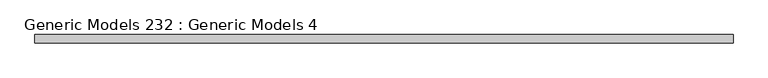
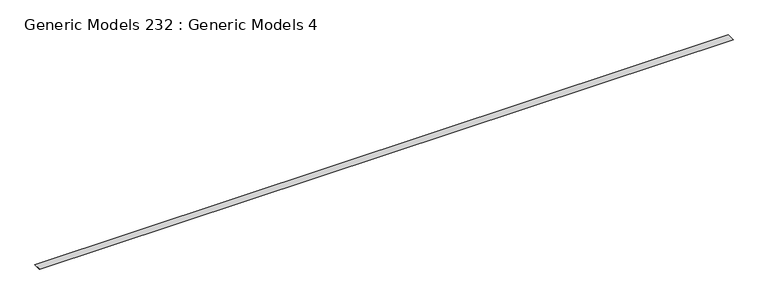
"""IFC4 building model written with IfcOpenShell, lengths in millimetres: proxy geometry, Generic Models 232 : Generic Models 4."""

import ifcopenshell
import ifcopenshell.guid

model = None  # the IFC model being written
_history = None  # IfcOwnerHistory: only IFC2X3 demands one
_inside = {}  # id of a spatial element -> (the spatial element, [elements in it])
_under = {}  # id of a project, library or spatial element -> (it, [spatial elements below it])
_declared = {}  # id of a project -> (the project, [libraries it declares])
_typed = {}  # id of a type object -> (the type object, [elements of that type])
_made_of = {}  # id of a material, layer set ... -> (it, [elements and type objects made of it])


def new_model(schema):
    """Start an empty IFC model of exactly this schema.

    Asked for "IFC4X3", IfcOpenShell would pick the latest addendum, in which some entities
    have other attributes; the version numbers below select the first issue.
    IFC2X3 requires an IfcOwnerHistory on every rooted entity: one is made here for all.
    """
    global model, _history
    if schema == "IFC4X3":
        model = ifcopenshell.file(schema_version=(4, 3, 0, 0))
    else:
        model = ifcopenshell.file(schema=schema)
    _inside.clear()
    _under.clear()
    _declared.clear()
    _typed.clear()
    _made_of.clear()
    _history = None
    if model.schema == "IFC2X3":
        org = make("IfcOrganization", Name="unknown")
        user = make(
            "IfcPersonAndOrganization",
            ThePerson=make("IfcPerson", FamilyName="unknown"),
            TheOrganization=org,
        )
        app = make(
            "IfcApplication",
            ApplicationDeveloper=org,
            Version="unknown",
            ApplicationFullName="unknown",
            ApplicationIdentifier="unknown",
        )
        _history = make(
            "IfcOwnerHistory",
            OwningUser=user,
            OwningApplication=app,
            ChangeAction="ADDED",
            CreationDate=0,
        )
    return model


def make(cls, **values):
    """One entity of the class cls with the attributes given. An attribute that is None is left unset."""
    return model.create_entity(
        cls, **{name: value for name, value in values.items() if value is not None}
    )


def rooted(cls, **values):
    """An entity with a GlobalId (a new one), such as an element, a storey or a relation."""
    return make(cls, GlobalId=ifcopenshell.guid.new(), OwnerHistory=_history, **values)


def si_unit(unit_type, name, prefix=None):
    """IfcSIUnit, for example si_unit("LENGTHUNIT", "METRE", prefix="MILLI")."""
    return make("IfcSIUnit", UnitType=unit_type, Prefix=prefix, Name=name)


def assignment(units):
    """IfcUnitAssignment: the units of a project."""
    return None if units is None else make("IfcUnitAssignment", Units=units)


def point(xyz):
    """IfcCartesianPoint."""
    return None if xyz is None else make("IfcCartesianPoint", Coordinates=xyz)


def direction(xyz):
    """IfcDirection."""
    return None if xyz is None else make("IfcDirection", DirectionRatios=xyz)


def frame(location, z_axis=None, x_axis=None):
    """IfcAxis2Placement3D, a coordinate frame: its origin and axes. An axis left out is left unset."""
    return make(
        "IfcAxis2Placement3D",
        Location=point(location),
        Axis=direction(z_axis),
        RefDirection=direction(x_axis),
    )


def origin():
    """The frame at (0, 0, 0) with its axes left unset."""
    return frame((0.0, 0.0, 0.0))


def place(relative_to, where):
    """IfcLocalPlacement: puts the frame where relative to a parent placement (None: the world)."""
    return make(
        "IfcLocalPlacement", PlacementRelTo=relative_to, RelativePlacement=where
    )


def context(
    kind, dimensions, precision=None, world=None, true_north=None, identifier=None
):
    """IfcGeometricRepresentationContext, for example the 3D "Model" context."""
    return make(
        "IfcGeometricRepresentationContext",
        ContextIdentifier=identifier,
        ContextType=kind,
        CoordinateSpaceDimension=dimensions,
        Precision=precision,
        WorldCoordinateSystem=world,
        TrueNorth=true_north,
    )


def project(units=None, contexts=None):
    """IfcProject with its units and contexts."""
    return rooted(
        "IfcProject",
        Name="project",
        RepresentationContexts=contexts,
        UnitsInContext=assignment(units),
    )


def spatial(cls, under=None, at=None, **own):
    """A site, building, storey or space (cls), placed at a placement, below another one or the project."""
    s = rooted(cls, ObjectPlacement=at, **own)
    if under is not None:
        _under.setdefault(under.id(), (under, []))[1].append(s)
    return s


def polyline(points):
    """IfcPolyline through the points."""
    return make("IfcPolyline", Points=[point(p) for p in points])


def outline(outer, holes=None, kind="AREA"):
    """IfcArbitraryClosedProfileDef: a profile drawn as a closed curve; with holes, ...WithVoids."""
    if holes is None:
        return make("IfcArbitraryClosedProfileDef", ProfileType=kind, OuterCurve=outer)
    return make(
        "IfcArbitraryProfileDefWithVoids",
        ProfileType=kind,
        OuterCurve=outer,
        InnerCurves=holes,
    )


def extrude(swept, where, along, depth):
    """IfcExtrudedAreaSolid: the profile swept, set in the frame where, extruded along a direction by depth."""
    return make(
        "IfcExtrudedAreaSolid",
        SweptArea=swept,
        Position=where,
        ExtrudedDirection=direction(along),
        Depth=depth,
    )


def shape(context_of_items, identifier, shape_type, items):
    """IfcShapeRepresentation: the items that make up one representation, for example the "Body"."""
    return make(
        "IfcShapeRepresentation",
        ContextOfItems=context_of_items,
        RepresentationIdentifier=identifier,
        RepresentationType=shape_type,
        Items=items,
    )


def source(mapping_origin, context_of_items, identifier, shape_type, items):
    """IfcRepresentationMap: a shape defined once, which mapped items show again and again."""
    return make(
        "IfcRepresentationMap",
        MappingOrigin=mapping_origin,
        MappedRepresentation=shape(context_of_items, identifier, shape_type, items),
    )


def transform(
    local_origin,
    x_axis=None,
    y_axis=None,
    z_axis=None,
    scale=None,
    scale2=None,
    scale3=None,
    uniform=True,
):
    """IfcCartesianTransformationOperator3D, or its non-uniform kind. x_axis, y_axis, z_axis: its Axis1, 2, 3."""
    if uniform:
        return make(
            "IfcCartesianTransformationOperator3D",
            Axis1=direction(x_axis),
            Axis2=direction(y_axis),
            LocalOrigin=point(local_origin),
            Scale=scale,
            Axis3=direction(z_axis),
        )
    return make(
        "IfcCartesianTransformationOperator3DnonUniform",
        Axis1=direction(x_axis),
        Axis2=direction(y_axis),
        LocalOrigin=point(local_origin),
        Scale=scale,
        Axis3=direction(z_axis),
        Scale2=scale2,
        Scale3=scale3,
    )


def mapped(mapping_source, mapping_target):
    """IfcMappedItem: shows the shape of a source again, moved by a transform."""
    return make(
        "IfcMappedItem", MappingSource=mapping_source, MappingTarget=mapping_target
    )


def made_of(thing, what):
    """Note that an element or type object is made of a material, layer set ...; save() writes the relation."""
    if what is not None:
        _made_of.setdefault(what.id(), (what, []))[1].append(thing)
    return thing


def element(
    cls,
    number,
    at=None,
    inside=None,
    cuts=None,
    type_object=None,
    material=None,
    context=None,
    identifier="Body",
    shape_type=None,
    held_by="IfcProductDefinitionShape",
    body=None,
    shapes=None,
    **own,
):
    """One element of the class cls, such as IfcWall. Its Tag is "e" and its number.

    at: its placement. inside: the storey or other place that contains it. cuts: it is an
    opening in that element (IfcRelVoidsElement). A single representation is given by context,
    identifier, shape_type and body (its items); several are given by shapes. held_by: the class
    of the entity that holds the representations. save() writes the other relations.
    """
    e = rooted(cls, Tag="e%d" % number, ObjectPlacement=at, **own)
    if body is not None:
        shapes = [shape(context, identifier, shape_type, body)]
    if shapes is not None:
        e.Representation = make(held_by, Representations=shapes)
    if inside is not None:
        _inside.setdefault(inside.id(), (inside, []))[1].append(e)
    if cuts is not None:
        rooted(
            "IfcRelVoidsElement", RelatingBuildingElement=cuts, RelatedOpeningElement=e
        )
    if type_object is not None:
        _typed.setdefault(type_object.id(), (type_object, []))[1].append(e)
    return made_of(e, material)


def aggregate(whole, parts):
    """IfcRelAggregates: a whole, such as a stair, and the parts it consists of."""
    return rooted("IfcRelAggregates", RelatingObject=whole, RelatedObjects=parts)


def save(model, path):
    """Write the relations noted so far, then the file.

    IfcRelAggregates (storeys below a building ...), IfcRelContainedInSpatialStructure (elements
    in a storey), IfcRelDefinesByType, IfcRelAssociatesMaterial and IfcRelDeclares: one each for
    every whole, place, type object, material and project.
    """
    for whole, parts in _under.values():
        aggregate(whole, parts)
    for where, things in _inside.values():
        rooted(
            "IfcRelContainedInSpatialStructure",
            RelatedElements=things,
            RelatingStructure=where,
        )
    for kind, things in _typed.values():
        rooted("IfcRelDefinesByType", RelatedObjects=things, RelatingType=kind)
    for what, things in _made_of.values():
        rooted("IfcRelAssociatesMaterial", RelatedObjects=things, RelatingMaterial=what)
    for by, libraries in _declared.values():
        rooted("IfcRelDeclares", RelatingContext=by, RelatedDefinitions=libraries)
    model.write(path)


def generic_models_232_generic_models_4_c391f1b5(model_context):
    return source(origin(), model_context, "Body", "SweptSolid", [
        extrude(outline(polyline([(11796.8702948, 127086.238344), (11763.5680231, 127103.3395105), (11988.322106, 127107.9460991), (11952.2508948, 127089.4230447), (11796.8702948, 127086.238344)])), frame((-10234.5171316, 0.0, 0.0), z_axis=(1.0, 0.0, 0.0), x_axis=(0.0, 1.0, 0.0)), (0.0, 0.0, 1.0), 18643.6),
    ])


if __name__ == "__main__":
    model = new_model("IFC4")
    model_context = context("Model", 3, world=origin())
    ifc_project = project(units=[si_unit("LENGTHUNIT", "METRE", prefix="MILLI")], contexts=[model_context])
    site = spatial("IfcSite", under=ifc_project)
    building = spatial("IfcBuilding", under=site)
    placement = place(None, origin())
    generic_models_232_generic_models_4_shape = generic_models_232_generic_models_4_c391f1b5(model_context)
    element("IfcBuildingElementProxy", 1, Name="Generic Models 232 : Generic Models 4", ObjectType="Generic Models 232 : Generic Models 4", at=placement, inside=building, context=model_context, shape_type="MappedRepresentation", body=[
        mapped(generic_models_232_generic_models_4_shape, transform((0.0, 0.0, 0.0), x_axis=(1.0, 0.0, 0.0), y_axis=(0.0, 1.0, 0.0), z_axis=(0.0, 0.0, 1.0))),
    ])
    save(model, "model.ifc")

# Revit data of these elements
# Element 1 (IfcBuildingElementProxy, "Generic Models 232 : Generic Models 4")
#   Materials on its faces: "_7/8\" SMOOTH TROWEL EXTERIOR STUCCO (COLOR PER OWNER) @ 2% SLOPE"
# Materials
#   "_7/8\" SMOOTH TROWEL EXTERIOR STUCCO (COLOR PER OWNER) @ 2% SLOPE": class "Generic", colour RGB 233 233 233, transparency 0, Cost = 0
